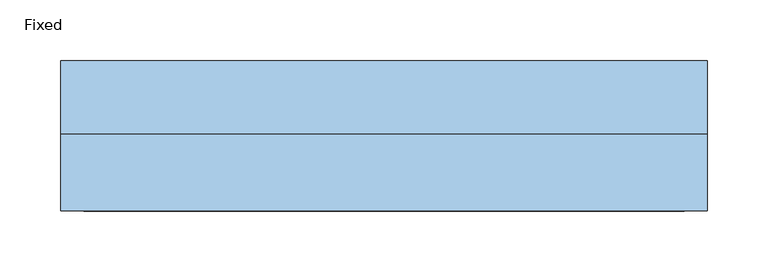
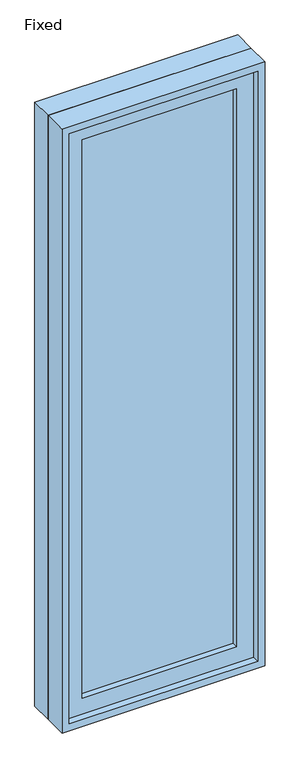
"""IFC4 building model written with IfcOpenShell, lengths in millimetres: window geometry, Fixed."""

from ifc_helpers import new_model, si_unit, frame, origin, place, context, project, spatial, polyline, outline, extrude, source, transform, mapped, element, save


def fixed_e4177030(model_context):
    return source(origin(), model_context, "Body", "SweptSolid", [
        extrude(outline(polyline([(165.1, -14.2875), (165.1, -26.9875), (-241.3, -26.9875), (-241.3, -14.2875), (165.1, -14.2875)])), frame((0.0, 0.0, 825.5), z_axis=(0.0, 0.0, 1.0), x_axis=(1.0, 0.0, 0.0)), (0.0, 0.0, 1.0), 1549.4),
        extrude(outline(polyline([(2419.35, -285.75), (781.05, -285.75), (781.05, 209.55), (2419.35, 209.55), (2419.35, -285.75)]), holes=[polyline([(2374.9, -241.3), (2374.9, 165.1), (825.5, 165.1), (825.5, -241.3), (2374.9, -241.3)])]), frame((0.0, -42.8625, 0.0), z_axis=(0.0, 1.0, 0.0), x_axis=(0.0, 0.0, 1.0)), (0.0, 0.0, 1.0), 44.45),
        extrude(outline(polyline([(2438.4, -304.8), (762.0, -304.8), (762.0, 228.6), (2438.4, 228.6), (2438.4, -304.8)]), holes=[polyline([(2406.65, -273.05), (2406.65, 196.85), (793.75, 196.85), (793.75, -273.05), (2406.65, -273.05)])]), frame((0.0, 1.5875, 0.0), z_axis=(0.0, 1.0, 0.0), x_axis=(0.0, 0.0, 1.0)), (0.0, 0.0, 1.0), 60.325),
        extrude(outline(polyline([(2438.4, 228.6), (2438.4, -304.8), (762.0, -304.8), (762.0, 228.6), (2438.4, 228.6)]), holes=[polyline([(2419.35, 209.55), (781.05, 209.55), (781.05, -285.75), (2419.35, -285.75), (2419.35, 209.55)])]), frame((0.0, -61.9125, 0.0), z_axis=(0.0, 1.0, 0.0), x_axis=(0.0, 0.0, 1.0)), (0.0, 0.0, 1.0), 63.5),
    ])


if __name__ == "__main__":
    model = new_model("IFC4")
    model_context = context("Model", 3, world=origin())
    ifc_project = project(units=[si_unit("LENGTHUNIT", "METRE", prefix="MILLI")], contexts=[model_context])
    site = spatial("IfcSite", under=ifc_project)
    building = spatial("IfcBuilding", under=site)
    placement = place(None, origin())
    fixed_shape = fixed_e4177030(model_context)
    element("IfcWindow", 1, ObjectType="Fixed : 66\" x 21\"  Screen", at=placement, inside=building, context=model_context, shape_type="MappedRepresentation", body=[
        mapped(fixed_shape, transform((0.0, 0.0, 0.0), x_axis=(1.0, 0.0, 0.0), y_axis=(0.0, 1.0, 0.0), z_axis=(0.0, 0.0, 1.0))),
    ])
    save(model, "model.ifc")

# Revit data of these elements
# Type "Fixed : 66\" x 21\"  Screen"
#   Type Mark = "70"
#   COBie.Type.CreatedBy = "doug.wood@us.ibm.com"
#   COBie.Type.CreatedOn = "2016-04-14T02:07:26"
#   COBie.Type.Name = "Windows_Fixed_66\" x 21\"  Screen_70"
#   COBie.Type.Category = "23-30 20 17 11 : Fixed Windows"
#   COBie.Type.Description = "Fixed_66\" x 21\"  Screen"
#   COBie.Type.Manufacturer = ""
#   COBie.Type.ModelNumber = ""
#   Construction Type Id = "GSP4R"
#   Assembly Code = "B2020100"
#   Analytic Construction = "1/8 in Pilkington single glazing"
#   COBie.Type.ReplacementCost = 0
#   Visual Light Transmittance = 0.9
#   Solar Heat Gain Coefficient = 0.78
#   Heat Transfer Coefficient (U) = 3.6886 W/(m²·K)
#   Height = 5' - 6"
#   Default Sill Height = 2' - 6"
#   Width = 1' - 9"
#   Window Inset = 0' - 0 3/4"
#   COBie.Type = no
#   Glass Pane Material = Screen
#   Sash Material = Sash - White
#   Wall Closure = (empty or 0)
# Element 1 (IfcWindow, "Fixed : 66\" x 21\"  Screen")
#   Materials on its faces: "Sash - White", "Screen"
# Materials
#   "Screen": class "Metal", colour RGB 120 120 120, transparency 0, Description = "Screen", Cost = 0
#   "Sash - White": class "Wood", colour RGB 255 255 255, transparency 0, Cost = 0
